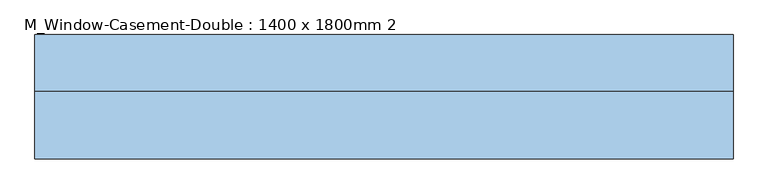
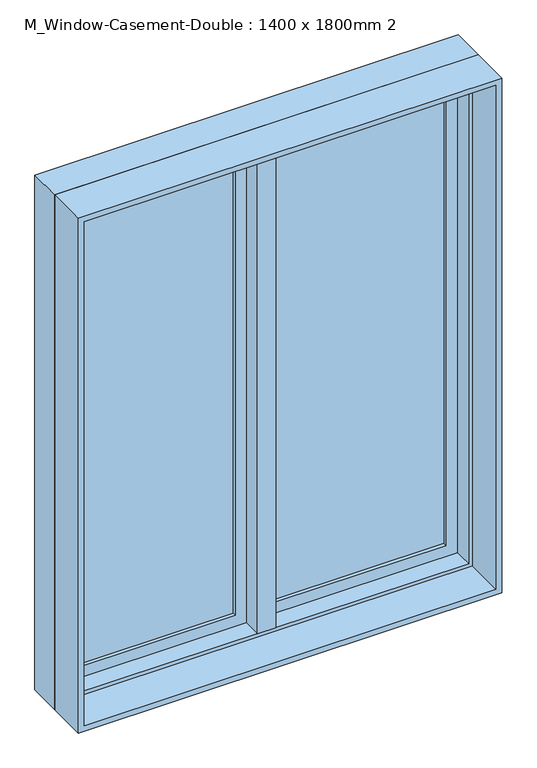
"""IFC4 building model written with IfcOpenShell, lengths in millimetres: window geometry, M_Window-Casement-Double : 1400 x 1800mm 2."""

from ifc_helpers import new_model, si_unit, frame, origin, place, context, project, spatial, polyline, outline, extrude, faceted_brep, source, transform, mapped, element, save


def m_window_casement_double_1400_x_1800mm_2_db642eaa(model_context):
    return source(origin(), model_context, "Body", "SolidModel", [
        faceted_brep([(9.525, 134.05, 2387.3), (-9.525, 134.05, 2387.3), (-9.525, 83.25, 2387.3), (9.525, 83.25, 2387.3), (9.525, 134.05, 612.7), (9.525, 83.25, 612.7), (-9.525, 83.25, 612.7), (-9.525, 134.05, 612.7), (-9.525, 83.25, 631.75), (-9.525, 83.25, 2368.25), (-30.1625, 83.25, 631.75), (-30.1625, 83.25, 2368.25), (-30.1625, 19.75, 631.75), (-30.1625, 19.75, 2368.25), (30.1625, 19.75, 631.75), (30.1625, 19.75, 2368.25), (30.1625, 83.25, 631.75), (30.1625, 83.25, 2368.25), (9.525, 83.25, 631.75), (9.525, 83.25, 2368.25)], [[[0, 1, 2, 3]], [[4, 5, 6, 7]], [[1, 0, 4, 7]], [[2, 1, 7, 6, 8, 9]], [[9, 8, 10, 11]], [[11, 10, 12, 13]], [[13, 12, 14, 15]], [[15, 14, 16, 17]], [[17, 16, 18, 19]], [[0, 3, 19, 18, 5, 4]], [[18, 8, 6, 5]], [[9, 19, 3, 2]], [[8, 18, 16, 14, 12, 10]], [[19, 9, 11, 13, 15, 17]]]),
        extrude(outline(polyline([(-66.675, 115.0), (-66.675, 108.65), (-630.15, 108.65), (-630.15, 115.0), (-66.675, 115.0)])), frame((0.0, 0.0, 669.85), z_axis=(0.0, 0.0, 1.0), x_axis=(1.0, 0.0, 0.0)), (0.0, 0.0, 1.0), 1660.3),
        extrude(outline(polyline([(-630.15, 95.95), (-630.15, 102.3), (-66.675, 102.3), (-66.675, 95.95), (-630.15, 95.95)])), frame((0.0, 0.0, 669.85), z_axis=(0.0, 0.0, 1.0), x_axis=(1.0, 0.0, 0.0)), (0.0, 0.0, 1.0), 1660.3),
        extrude(outline(polyline([(630.15, 115.0), (630.15, 108.65), (66.675, 108.65), (66.675, 115.0), (630.15, 115.0)])), frame((0.0, 0.0, 669.85), z_axis=(0.0, 0.0, 1.0), x_axis=(1.0, 0.0, 0.0)), (0.0, 0.0, 1.0), 1660.3),
        extrude(outline(polyline([(66.675, 95.95), (66.675, 102.3), (630.15, 102.3), (630.15, 95.95), (66.675, 95.95)])), frame((0.0, 0.0, 669.85), z_axis=(0.0, 0.0, 1.0), x_axis=(1.0, 0.0, 0.0)), (0.0, 0.0, 1.0), 1660.3),
        extrude(outline(polyline([(2387.3, -687.3), (612.7, -687.3), (612.7, -9.525), (2387.3, -9.525), (2387.3, -687.3)]), holes=[polyline([(2330.15, -66.675), (669.85, -66.675), (669.85, -630.15), (2330.15, -630.15), (2330.15, -66.675)])]), frame((0.0, 83.25, 0.0), z_axis=(0.0, 1.0, 0.0), x_axis=(0.0, 0.0, 1.0)), (0.0, 0.0, 1.0), 44.45),
        extrude(outline(polyline([(612.7, 687.3), (2387.3, 687.3), (2387.3, 9.525), (612.7, 9.525), (612.7, 687.3)]), holes=[polyline([(669.85, 66.675), (2330.15, 66.675), (2330.15, 630.15), (669.85, 630.15), (669.85, 66.675)])]), frame((0.0, 83.25, 0.0), z_axis=(0.0, 1.0, 0.0), x_axis=(0.0, 0.0, 1.0)), (0.0, 0.0, 1.0), 44.45),
        extrude(outline(polyline([(2400.0, -700.0), (600.0, -700.0), (600.0, 700.0), (2400.0, 700.0), (2400.0, -700.0)]), holes=[polyline([(2380.95, 680.95), (619.05, 680.95), (619.05, -680.95), (2380.95, -680.95), (2380.95, 680.95)])]), frame((0.0, -115.0, 0.0), z_axis=(0.0, 1.0, 0.0), x_axis=(0.0, 0.0, 1.0)), (0.0, 0.0, 1.0), 134.75),
        faceted_brep([(668.25, 83.25, 2368.25), (668.25, 19.75, 2368.25), (-668.25, 19.75, 2368.25), (-668.25, 83.25, 2368.25), (687.3, 134.05, 2387.3), (687.3, 83.25, 2387.3), (-687.3, 83.25, 2387.3), (-687.3, 134.05, 2387.3), (700.0, 19.75, 2400.0), (700.0, 134.05, 2400.0), (-700.0, 134.05, 2400.0), (-700.0, 19.75, 2400.0), (-668.25, 19.75, 631.75), (-668.25, 83.25, 631.75), (-687.3, 83.25, 612.7), (-687.3, 134.05, 612.7), (-700.0, 134.05, 600.0), (-700.0, 19.75, 600.0), (668.25, 19.75, 631.75), (668.25, 83.25, 631.75), (687.3, 83.25, 612.7), (687.3, 134.05, 612.7), (700.0, 134.05, 600.0), (700.0, 19.75, 600.0)], [[[0, 1, 2, 3]], [[4, 5, 6, 7]], [[8, 9, 10, 11]], [[3, 2, 12, 13]], [[7, 6, 14, 15]], [[11, 10, 16, 17]], [[13, 12, 18, 19]], [[15, 14, 20, 21]], [[17, 16, 22, 23]], [[11, 17, 23, 8], [1, 18, 12, 2]], [[19, 18, 1, 0]], [[5, 20, 14, 6], [3, 13, 19, 0]], [[21, 20, 5, 4]], [[23, 22, 9, 8]], [[9, 22, 16, 10], [7, 15, 21, 4]]]),
    ])


if __name__ == "__main__":
    model = new_model("IFC4")
    model_context = context("Model", 3, world=origin())
    ifc_project = project(units=[si_unit("LENGTHUNIT", "METRE", prefix="MILLI")], contexts=[model_context])
    site = spatial("IfcSite", under=ifc_project)
    building = spatial("IfcBuilding", under=site)
    placement = place(None, origin())
    m_window_casement_double_1400_x_1800mm_2_shape = m_window_casement_double_1400_x_1800mm_2_db642eaa(model_context)
    element("IfcWindow", 1, ObjectType="M_Window-Casement-Double : 1400 x 1800mm 2", at=placement, inside=building, context=model_context, shape_type="MappedRepresentation", body=[
        mapped(m_window_casement_double_1400_x_1800mm_2_shape, transform((0.0, 0.0, 0.0), x_axis=(1.0, 0.0, 0.0), y_axis=(0.0, 1.0, 0.0), z_axis=(0.0, 0.0, 1.0))),
    ])
    save(model, "model.ifc")

# Revit data of these elements
# Type "M_Window-Casement-Double : 1400 x 1800mm 2"
#   Type Mark = "27"
#   Fire Rating = "0.5h"
#   Assembly Code = "B2020100"
#   Analytic Construction = "Double glazing - domestic"
#   Frame Extension [instance default] = 0.635 cm
#   Window Inset [instance default] = 0 cm
#   Wall Thickness [instance default] = 15 cm
#   Interior Wall Closure [instance default] = 5.475 cm
#   Half Width = 70 cm
#   Visual Light Transmittance = 0.81
#   Thermal Resistance (R) = 0.319569 (m²·K)/W
#   Solar Heat Gain Coefficient = 0.76
#   Rough Width = 141.5 cm
#   Rough Height = 181.5 cm
#   Height = 180 cm
#   Heat Transfer Coefficient (U) = 3.12929 W/(m²·K)
#   Exterior Wall Closure [instance default] = 3.18 cm
#   Extension Jamb [instance default] = 5.475 cm
#   Default Sill Height = 60 cm
#   Width = 140 cm
#   Muntin Visibility = yes
#   Interior Trim Visibility [instance default] = yes
#   Exterior Trim Visibility [instance default] = yes
#   Extension Jamb Visibility [instance default] = yes
#   Interior Trim Material = Wood - Stained
#   Muntin Pattern = M_Muntin Pattern_2x2 : M_Muntin Pattern_2x2
#   Interior Trim = M_Trim-Window-Interior-Flat : Picture Frame
#   Interior Frame Material = Wood - Stained
#   Glass Panel Material = Glass
#   Exterior Trim Material = Clad - White
#   Exterior Trim = M_Trim-Window-Exterior-Flat : with Sill
#   Exterior Frame Material = Clad - White
#   Wall Closure = (empty or 0)
# Element 1 (IfcWindow, "M_Window-Casement-Double : 1400 x 1800mm 2")
#   Wall Thickness = 23 cm
#   Extension Jamb = 13.475 cm
#   Materials on its faces: "Wood - Stained", "Glass", "Clad - White"
# Materials
#   "Wood - Stained": class "Wood", colour RGB 224 178 126, transparency 0, Cost = 0
#   "Glass": class "Glass", colour RGB 0 128 192, transparency 0.9, Description = "Soda Lime Glass", Cost = 0
#   "Clad - White": class "Wood", colour RGB 242 242 238, transparency 0, Cost = 0
